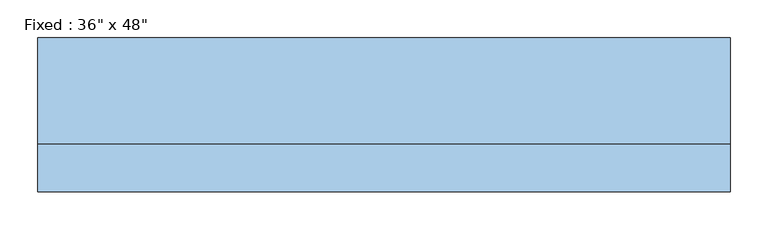
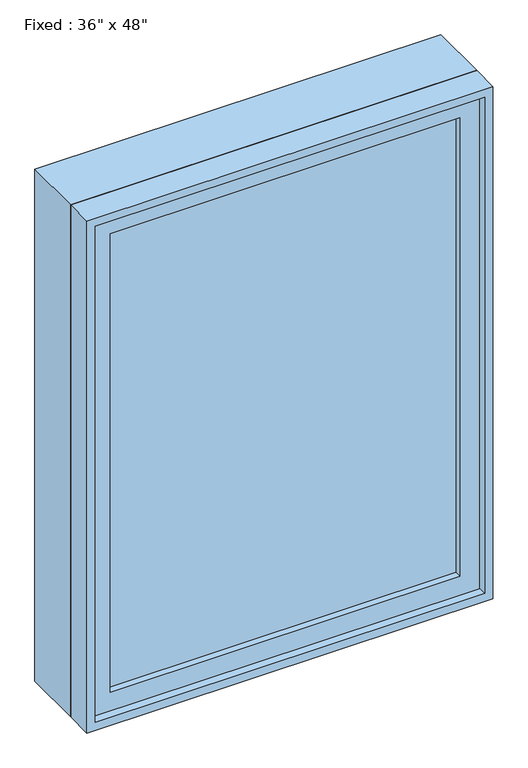
"""IFC4 building model written with IfcOpenShell, lengths in millimetres: window geometry."""

import ifcopenshell
import ifcopenshell.guid

model = None  # the IFC model being written
_history = None  # IfcOwnerHistory: only IFC2X3 demands one
_inside = {}  # id of a spatial element -> (the spatial element, [elements in it])
_under = {}  # id of a project, library or spatial element -> (it, [spatial elements below it])
_declared = {}  # id of a project -> (the project, [libraries it declares])
_typed = {}  # id of a type object -> (the type object, [elements of that type])
_made_of = {}  # id of a material, layer set ... -> (it, [elements and type objects made of it])


def new_model(schema):
    """Start an empty IFC model of exactly this schema.

    Asked for "IFC4X3", IfcOpenShell would pick the latest addendum, in which some entities
    have other attributes; the version numbers below select the first issue.
    IFC2X3 requires an IfcOwnerHistory on every rooted entity: one is made here for all.
    """
    global model, _history
    if schema == "IFC4X3":
        model = ifcopenshell.file(schema_version=(4, 3, 0, 0))
    else:
        model = ifcopenshell.file(schema=schema)
    _inside.clear()
    _under.clear()
    _declared.clear()
    _typed.clear()
    _made_of.clear()
    _history = None
    if model.schema == "IFC2X3":
        org = make("IfcOrganization", Name="unknown")
        user = make(
            "IfcPersonAndOrganization",
            ThePerson=make("IfcPerson", FamilyName="unknown"),
            TheOrganization=org,
        )
        app = make(
            "IfcApplication",
            ApplicationDeveloper=org,
            Version="unknown",
            ApplicationFullName="unknown",
            ApplicationIdentifier="unknown",
        )
        _history = make(
            "IfcOwnerHistory",
            OwningUser=user,
            OwningApplication=app,
            ChangeAction="ADDED",
            CreationDate=0,
        )
    return model


def make(cls, **values):
    """One entity of the class cls with the attributes given. An attribute that is None is left unset."""
    return model.create_entity(
        cls, **{name: value for name, value in values.items() if value is not None}
    )


def rooted(cls, **values):
    """An entity with a GlobalId (a new one), such as an element, a storey or a relation."""
    return make(cls, GlobalId=ifcopenshell.guid.new(), OwnerHistory=_history, **values)


def si_unit(unit_type, name, prefix=None):
    """IfcSIUnit, for example si_unit("LENGTHUNIT", "METRE", prefix="MILLI")."""
    return make("IfcSIUnit", UnitType=unit_type, Prefix=prefix, Name=name)


def assignment(units):
    """IfcUnitAssignment: the units of a project."""
    return None if units is None else make("IfcUnitAssignment", Units=units)


def point(xyz):
    """IfcCartesianPoint."""
    return None if xyz is None else make("IfcCartesianPoint", Coordinates=xyz)


def direction(xyz):
    """IfcDirection."""
    return None if xyz is None else make("IfcDirection", DirectionRatios=xyz)


def frame(location, z_axis=None, x_axis=None):
    """IfcAxis2Placement3D, a coordinate frame: its origin and axes. An axis left out is left unset."""
    return make(
        "IfcAxis2Placement3D",
        Location=point(location),
        Axis=direction(z_axis),
        RefDirection=direction(x_axis),
    )


def origin():
    """The frame at (0, 0, 0) with its axes left unset."""
    return frame((0.0, 0.0, 0.0))


def place(relative_to, where):
    """IfcLocalPlacement: puts the frame where relative to a parent placement (None: the world)."""
    return make(
        "IfcLocalPlacement", PlacementRelTo=relative_to, RelativePlacement=where
    )


def context(
    kind, dimensions, precision=None, world=None, true_north=None, identifier=None
):
    """IfcGeometricRepresentationContext, for example the 3D "Model" context."""
    return make(
        "IfcGeometricRepresentationContext",
        ContextIdentifier=identifier,
        ContextType=kind,
        CoordinateSpaceDimension=dimensions,
        Precision=precision,
        WorldCoordinateSystem=world,
        TrueNorth=true_north,
    )


def project(units=None, contexts=None):
    """IfcProject with its units and contexts."""
    return rooted(
        "IfcProject",
        Name="project",
        RepresentationContexts=contexts,
        UnitsInContext=assignment(units),
    )


def spatial(cls, under=None, at=None, **own):
    """A site, building, storey or space (cls), placed at a placement, below another one or the project."""
    s = rooted(cls, ObjectPlacement=at, **own)
    if under is not None:
        _under.setdefault(under.id(), (under, []))[1].append(s)
    return s


def polyline(points):
    """IfcPolyline through the points."""
    return make("IfcPolyline", Points=[point(p) for p in points])


def outline(outer, holes=None, kind="AREA"):
    """IfcArbitraryClosedProfileDef: a profile drawn as a closed curve; with holes, ...WithVoids."""
    if holes is None:
        return make("IfcArbitraryClosedProfileDef", ProfileType=kind, OuterCurve=outer)
    return make(
        "IfcArbitraryProfileDefWithVoids",
        ProfileType=kind,
        OuterCurve=outer,
        InnerCurves=holes,
    )


def extrude(swept, where, along, depth):
    """IfcExtrudedAreaSolid: the profile swept, set in the frame where, extruded along a direction by depth."""
    return make(
        "IfcExtrudedAreaSolid",
        SweptArea=swept,
        Position=where,
        ExtrudedDirection=direction(along),
        Depth=depth,
    )


def shape(context_of_items, identifier, shape_type, items):
    """IfcShapeRepresentation: the items that make up one representation, for example the "Body"."""
    return make(
        "IfcShapeRepresentation",
        ContextOfItems=context_of_items,
        RepresentationIdentifier=identifier,
        RepresentationType=shape_type,
        Items=items,
    )


def source(mapping_origin, context_of_items, identifier, shape_type, items):
    """IfcRepresentationMap: a shape defined once, which mapped items show again and again."""
    return make(
        "IfcRepresentationMap",
        MappingOrigin=mapping_origin,
        MappedRepresentation=shape(context_of_items, identifier, shape_type, items),
    )


def transform(
    local_origin,
    x_axis=None,
    y_axis=None,
    z_axis=None,
    scale=None,
    scale2=None,
    scale3=None,
    uniform=True,
):
    """IfcCartesianTransformationOperator3D, or its non-uniform kind. x_axis, y_axis, z_axis: its Axis1, 2, 3."""
    if uniform:
        return make(
            "IfcCartesianTransformationOperator3D",
            Axis1=direction(x_axis),
            Axis2=direction(y_axis),
            LocalOrigin=point(local_origin),
            Scale=scale,
            Axis3=direction(z_axis),
        )
    return make(
        "IfcCartesianTransformationOperator3DnonUniform",
        Axis1=direction(x_axis),
        Axis2=direction(y_axis),
        LocalOrigin=point(local_origin),
        Scale=scale,
        Axis3=direction(z_axis),
        Scale2=scale2,
        Scale3=scale3,
    )


def mapped(mapping_source, mapping_target):
    """IfcMappedItem: shows the shape of a source again, moved by a transform."""
    return make(
        "IfcMappedItem", MappingSource=mapping_source, MappingTarget=mapping_target
    )


def made_of(thing, what):
    """Note that an element or type object is made of a material, layer set ...; save() writes the relation."""
    if what is not None:
        _made_of.setdefault(what.id(), (what, []))[1].append(thing)
    return thing


def element(
    cls,
    number,
    at=None,
    inside=None,
    cuts=None,
    type_object=None,
    material=None,
    context=None,
    identifier="Body",
    shape_type=None,
    held_by="IfcProductDefinitionShape",
    body=None,
    shapes=None,
    **own,
):
    """One element of the class cls, such as IfcWall. Its Tag is "e" and its number.

    at: its placement. inside: the storey or other place that contains it. cuts: it is an
    opening in that element (IfcRelVoidsElement). A single representation is given by context,
    identifier, shape_type and body (its items); several are given by shapes. held_by: the class
    of the entity that holds the representations. save() writes the other relations.
    """
    e = rooted(cls, Tag="e%d" % number, ObjectPlacement=at, **own)
    if body is not None:
        shapes = [shape(context, identifier, shape_type, body)]
    if shapes is not None:
        e.Representation = make(held_by, Representations=shapes)
    if inside is not None:
        _inside.setdefault(inside.id(), (inside, []))[1].append(e)
    if cuts is not None:
        rooted(
            "IfcRelVoidsElement", RelatingBuildingElement=cuts, RelatedOpeningElement=e
        )
    if type_object is not None:
        _typed.setdefault(type_object.id(), (type_object, []))[1].append(e)
    return made_of(e, material)


def aggregate(whole, parts):
    """IfcRelAggregates: a whole, such as a stair, and the parts it consists of."""
    return rooted("IfcRelAggregates", RelatingObject=whole, RelatedObjects=parts)


def save(model, path):
    """Write the relations noted so far, then the file.

    IfcRelAggregates (storeys below a building ...), IfcRelContainedInSpatialStructure (elements
    in a storey), IfcRelDefinesByType, IfcRelAssociatesMaterial and IfcRelDeclares: one each for
    every whole, place, type object, material and project.
    """
    for whole, parts in _under.values():
        aggregate(whole, parts)
    for where, things in _inside.values():
        rooted(
            "IfcRelContainedInSpatialStructure",
            RelatedElements=things,
            RelatingStructure=where,
        )
    for kind, things in _typed.values():
        rooted("IfcRelDefinesByType", RelatedObjects=things, RelatingType=kind)
    for what, things in _made_of.values():
        rooted("IfcRelAssociatesMaterial", RelatedObjects=things, RelatingMaterial=what)
    for by, libraries in _declared.values():
        rooted("IfcRelDeclares", RelatingContext=by, RelatedDefinitions=libraries)
    model.write(path)


def window_209efcd5(model_context):
    return source(origin(), model_context, "Body", "SweptSolid", [
        extrude(outline(polyline([(355.6, -53.975), (355.6, -66.675), (-431.8, -66.675), (-431.8, -53.975), (355.6, -53.975)])), frame((0.0, 0.0, 977.9), z_axis=(0.0, 0.0, 1.0), x_axis=(1.0, 0.0, 0.0)), (0.0, 0.0, 1.0), 1092.2),
        extrude(outline(polyline([(2114.55, -476.25), (933.45, -476.25), (933.45, 400.05), (2114.55, 400.05), (2114.55, -476.25)]), holes=[polyline([(2070.1, -431.8), (2070.1, 355.6), (977.9, 355.6), (977.9, -431.8), (2070.1, -431.8)])]), frame((0.0, -82.55, 0.0), z_axis=(0.0, 1.0, 0.0), x_axis=(0.0, 0.0, 1.0)), (0.0, 0.0, 1.0), 44.45),
        extrude(outline(polyline([(2133.6, -495.3), (914.4, -495.3), (914.4, 419.1), (2133.6, 419.1), (2133.6, -495.3)]), holes=[polyline([(2101.85, -463.55), (2101.85, 387.35), (946.15, 387.35), (946.15, -463.55), (2101.85, -463.55)])]), frame((0.0, -38.1, 0.0), z_axis=(0.0, 1.0, 0.0), x_axis=(0.0, 0.0, 1.0)), (0.0, 0.0, 1.0), 139.7),
        extrude(outline(polyline([(2133.6, 419.1), (2133.6, -495.3), (914.4, -495.3), (914.4, 419.1), (2133.6, 419.1)]), holes=[polyline([(2114.55, 400.05), (933.45, 400.05), (933.45, -476.25), (2114.55, -476.25), (2114.55, 400.05)])]), frame((0.0, -101.6, 0.0), z_axis=(0.0, 1.0, 0.0), x_axis=(0.0, 0.0, 1.0)), (0.0, 0.0, 1.0), 63.5),
    ])


if __name__ == "__main__":
    model = new_model("IFC4")
    model_context = context("Model", 3, world=origin())
    ifc_project = project(units=[si_unit("LENGTHUNIT", "METRE", prefix="MILLI")], contexts=[model_context])
    site = spatial("IfcSite", under=ifc_project)
    building = spatial("IfcBuilding", under=site)
    placement = place(None, origin())
    window_shape = window_209efcd5(model_context)
    element("IfcWindow", 1, ObjectType="Fixed : 36\" x 48\"", at=placement, inside=building, context=model_context, shape_type="MappedRepresentation", body=[
        mapped(window_shape, transform((0.0, 0.0, 0.0), x_axis=(1.0, 0.0, 0.0), y_axis=(0.0, 1.0, 0.0), z_axis=(0.0, 0.0, 1.0))),
    ])
    save(model, "model.ifc")

# Revit data of these elements
# Project information
#   Project Issue Date = "Issue Date"
#   Project Status = "Project Status"
#   Client Name = "Owner"
#   Project Address = "Enter address here"
#   Project Name = "Project Name"
#   Project Number = "Project Number"
# Type "Fixed : 36\" x 48\""
#   Type Mark = "1"
#   Construction Type Id = "GSP4R"
#   Assembly Code = "B2020100"
#   Analytic Construction = "1/8 in Pilkington single glazing"
#   Visual Light Transmittance = 0.9
#   Solar Heat Gain Coefficient = 0.78
#   Heat Transfer Coefficient (U) = 0.6496 BTU/(h·ft²·°F)
#   Height = 4' - 0"
#   Default Sill Height = 3' - 0"
#   Width = 3' - 0"
#   Window Inset = 0' - 0 3/4"
#   Define Thermal Properties by = 1
#   Define Thermal Properties by = 1
#   Glass Pane Material = Glass
#   Sash Material = Sash
#   Wall Closure = (empty or 0)
# Element 1 (IfcWindow, "Fixed : 36\" x 48\"")
#   Materials on its faces: "Sash", "Glass"
# Materials
#   "Glass": class "Glass", colour RGB 0 128 192, transparency 0.75, Description = "Soda Lime Glass", Cost = 0
#   "Sash": class "Wood", colour RGB 224 178 126, transparency 0, Cost = 0
